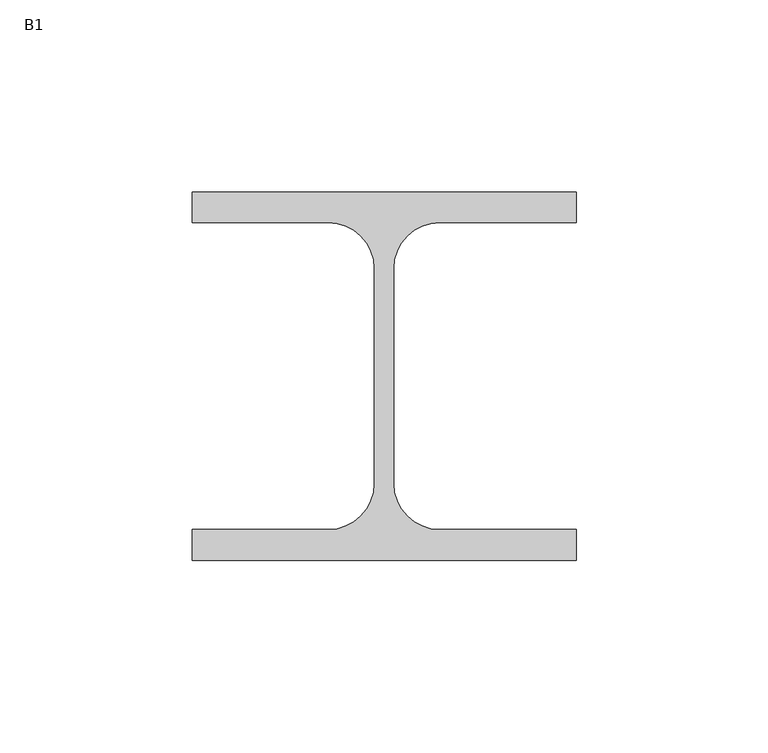
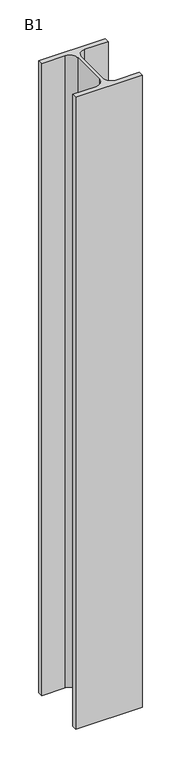
"""IFC4 building model written with IfcOpenShell, lengths in millimetres: proxy geometry, B1."""

from ifc_helpers import new_model, si_unit, point, frame_2d, origin, origin_with_axes, place, context, project, spatial, polyline, circle_curve, trimmed, segment, composite_curve, outline, extrude, source, transform, mapped, element, save


def b1_5aaa9024(model_context):
    return source(origin(), model_context, "Body", "SweptSolid", [
        extrude(outline(composite_curve([segment(polyline([(50.0, 48.0), (50.0, 40.0), (14.5, 40.0)]), True, "CONTINUOUS"), segment(trimmed(circle_curve(frame_2d((14.5, 28.0)), 12.0), [point((14.5, 40.0))], [point((2.5, 28.0))], True, "CARTESIAN"), True, "CONTINUOUS"), segment(polyline([(2.5, 28.0), (2.5, -28.0)]), True, "CONTINUOUS"), segment(trimmed(circle_curve(frame_2d((14.5, -28.0)), 12.0), [point((2.5, -28.0))], [point((14.5, -40.0))], True, "CARTESIAN"), True, "CONTINUOUS"), segment(polyline([(14.5, -40.0), (50.0, -40.0), (50.0, -48.0), (-50.0, -48.0), (-50.0, -40.0), (-14.5, -40.0)]), True, "CONTINUOUS"), segment(trimmed(circle_curve(frame_2d((-14.5, -28.0)), 12.0), [point((-14.5, -40.0))], [point((-2.5, -28.0))], True, "CARTESIAN"), True, "CONTINUOUS"), segment(polyline([(-2.5, -28.0), (-2.5, 28.0)]), True, "CONTINUOUS"), segment(trimmed(circle_curve(frame_2d((-14.5, 28.0)), 12.0), [point((-2.5, 28.0))], [point((-14.5, 40.0))], True, "CARTESIAN"), True, "CONTINUOUS"), segment(polyline([(-14.5, 40.0), (-50.0, 40.0), (-50.0, 48.0), (50.0, 48.0)]), True, "CONTINUOUS")], self_intersect=False)), origin_with_axes(), (0.0, 0.0, 1.0), 1000.0),
    ])


if __name__ == "__main__":
    model = new_model("IFC4")
    model_context = context("Model", 3, world=origin())
    ifc_project = project(units=[si_unit("LENGTHUNIT", "METRE", prefix="MILLI")], contexts=[model_context])
    site = spatial("IfcSite", under=ifc_project)
    building = spatial("IfcBuilding", under=site)
    placement = place(None, origin())
    b1_shape = b1_5aaa9024(model_context)
    element("IfcBuildingElementProxy", 1, Name="B1", ObjectType="B1", at=placement, inside=building, context=model_context, shape_type="MappedRepresentation", body=[
        mapped(b1_shape, transform((0.0, 0.0, 0.0), x_axis=(1.0, 0.0, 0.0), y_axis=(0.0, 1.0, 0.0), z_axis=(0.0, 0.0, 1.0))),
    ])
    save(model, "model.ifc")

# Revit data of these elements
# Project information
#   IfcSite GUID = "2K22w_rODEpOB_Z07mSHTM"
#   IfcBuilding GUID = "1$FKhNmbrE7fPtvvYM13W8"
#   IfcProject GUID = "3$9OzLmxr8buAEbGOTnNWo"
#   IfcDecomposes = "My Project"
#   IfcDecomposesGUID = "3$9OzLmxr8buAEbGOTnNWo"
#   BuildingName = "Building A"
#   SiteName = "My Site"
#   IfcProject Name = "My Project"
#   Original IFC File Name = "C:\\Users\\Jonathan\\Documents\\GitHub\\building.py\\model.ifc"
#   Original IFC File Size = "2436"
#   Revit File Last Updated = "638435876807059664"
#   Revit Importer Version = "Importer 24.2.0.63"
#   Import Method = "Hybrid"
#   Project Issue Date = "Issue Date"
#   Project Status = "Project Status"
#   Client Name = "Owner"
#   Project Address = "Enter address here"
#   Project Name = "Project Name"
#   Project Number = "Project Number"
